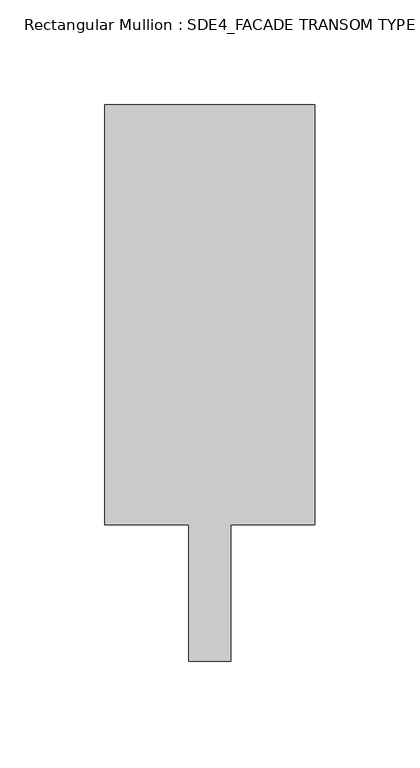
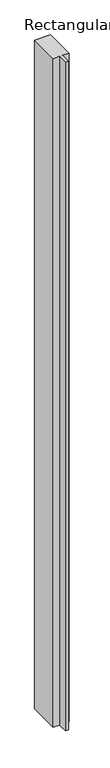
"""IFC4 building model written with IfcOpenShell, lengths in millimetres: member geometry, Rectangular Mullion : SDE4_FACADE TRANSOM TYPE 2."""

from ifc_helpers import new_model, si_unit, frame, origin, place, context, project, spatial, polyline, outline, extrude, source, transform, mapped, element, save


def rectangular_mullion_sde4_facade_transom_type_2_7f01d7f2(model_context):
    return source(origin(), model_context, "Body", "SweptSolid", [
        extrude(outline(polyline([(50.0, 132.5), (50.0, -67.5), (10.0, -67.5), (10.0, -132.5), (-10.0, -132.5), (-10.0, -67.5), (-50.0, -67.5), (-50.0, 132.5), (50.0, 132.5)])), frame((0.0, 0.0, -4423.1142131), z_axis=(0.0, 0.0, 1.0), x_axis=(1.0, 0.0, 0.0)), (0.0, 0.0, 1.0), 4423.1142131),
    ])


if __name__ == "__main__":
    model = new_model("IFC4")
    model_context = context("Model", 3, world=origin())
    ifc_project = project(units=[si_unit("LENGTHUNIT", "METRE", prefix="MILLI")], contexts=[model_context])
    site = spatial("IfcSite", under=ifc_project)
    building = spatial("IfcBuilding", under=site)
    placement = place(None, origin())
    rectangular_mullion_sde4_facade_transom_type_2_shape = rectangular_mullion_sde4_facade_transom_type_2_7f01d7f2(model_context)
    element("IfcMember", 1, ObjectType="Rectangular Mullion : SDE4_FACADE TRANSOM TYPE 2", at=placement, inside=building, context=model_context, shape_type="MappedRepresentation", body=[
        mapped(rectangular_mullion_sde4_facade_transom_type_2_shape, transform((0.0, 0.0, 0.0), x_axis=(1.0, 0.0, 0.0), y_axis=(0.0, 1.0, 0.0), z_axis=(0.0, 0.0, 1.0))),
    ])
    save(model, "model.ifc")

# Revit data of these elements
# Type "Rectangular Mullion : SDE4_FACADE TRANSOM TYPE 2"
#   built-in parameter 1007322 = 0.869423 (stored number, unit not read)
#   built-in parameter 1007321 = 0.164042 (stored number, unit not read)
#   built-in parameter 1007320 = 0.164042 (stored number, unit not read)
